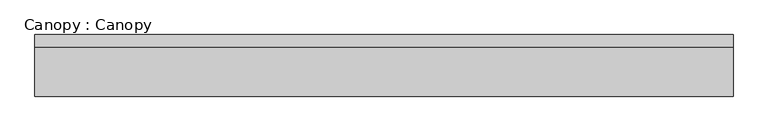
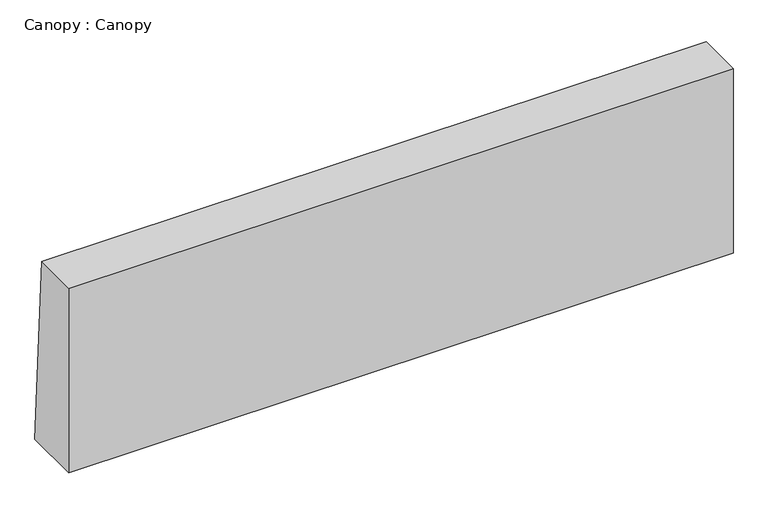
"""IFC4 building model written with IfcOpenShell, lengths in millimetres: proxy geometry, Canopy : Canopy."""

import ifcopenshell
import ifcopenshell.guid

model = None  # the IFC model being written
_history = None  # IfcOwnerHistory: only IFC2X3 demands one
_inside = {}  # id of a spatial element -> (the spatial element, [elements in it])
_under = {}  # id of a project, library or spatial element -> (it, [spatial elements below it])
_declared = {}  # id of a project -> (the project, [libraries it declares])
_typed = {}  # id of a type object -> (the type object, [elements of that type])
_made_of = {}  # id of a material, layer set ... -> (it, [elements and type objects made of it])


def new_model(schema):
    """Start an empty IFC model of exactly this schema.

    Asked for "IFC4X3", IfcOpenShell would pick the latest addendum, in which some entities
    have other attributes; the version numbers below select the first issue.
    IFC2X3 requires an IfcOwnerHistory on every rooted entity: one is made here for all.
    """
    global model, _history
    if schema == "IFC4X3":
        model = ifcopenshell.file(schema_version=(4, 3, 0, 0))
    else:
        model = ifcopenshell.file(schema=schema)
    _inside.clear()
    _under.clear()
    _declared.clear()
    _typed.clear()
    _made_of.clear()
    _history = None
    if model.schema == "IFC2X3":
        org = make("IfcOrganization", Name="unknown")
        user = make(
            "IfcPersonAndOrganization",
            ThePerson=make("IfcPerson", FamilyName="unknown"),
            TheOrganization=org,
        )
        app = make(
            "IfcApplication",
            ApplicationDeveloper=org,
            Version="unknown",
            ApplicationFullName="unknown",
            ApplicationIdentifier="unknown",
        )
        _history = make(
            "IfcOwnerHistory",
            OwningUser=user,
            OwningApplication=app,
            ChangeAction="ADDED",
            CreationDate=0,
        )
    return model


def make(cls, **values):
    """One entity of the class cls with the attributes given. An attribute that is None is left unset."""
    return model.create_entity(
        cls, **{name: value for name, value in values.items() if value is not None}
    )


def rooted(cls, **values):
    """An entity with a GlobalId (a new one), such as an element, a storey or a relation."""
    return make(cls, GlobalId=ifcopenshell.guid.new(), OwnerHistory=_history, **values)


def si_unit(unit_type, name, prefix=None):
    """IfcSIUnit, for example si_unit("LENGTHUNIT", "METRE", prefix="MILLI")."""
    return make("IfcSIUnit", UnitType=unit_type, Prefix=prefix, Name=name)


def assignment(units):
    """IfcUnitAssignment: the units of a project."""
    return None if units is None else make("IfcUnitAssignment", Units=units)


def point(xyz):
    """IfcCartesianPoint."""
    return None if xyz is None else make("IfcCartesianPoint", Coordinates=xyz)


def direction(xyz):
    """IfcDirection."""
    return None if xyz is None else make("IfcDirection", DirectionRatios=xyz)


def frame(location, z_axis=None, x_axis=None):
    """IfcAxis2Placement3D, a coordinate frame: its origin and axes. An axis left out is left unset."""
    return make(
        "IfcAxis2Placement3D",
        Location=point(location),
        Axis=direction(z_axis),
        RefDirection=direction(x_axis),
    )


def origin():
    """The frame at (0, 0, 0) with its axes left unset."""
    return frame((0.0, 0.0, 0.0))


def place(relative_to, where):
    """IfcLocalPlacement: puts the frame where relative to a parent placement (None: the world)."""
    return make(
        "IfcLocalPlacement", PlacementRelTo=relative_to, RelativePlacement=where
    )


def context(
    kind, dimensions, precision=None, world=None, true_north=None, identifier=None
):
    """IfcGeometricRepresentationContext, for example the 3D "Model" context."""
    return make(
        "IfcGeometricRepresentationContext",
        ContextIdentifier=identifier,
        ContextType=kind,
        CoordinateSpaceDimension=dimensions,
        Precision=precision,
        WorldCoordinateSystem=world,
        TrueNorth=true_north,
    )


def project(units=None, contexts=None):
    """IfcProject with its units and contexts."""
    return rooted(
        "IfcProject",
        Name="project",
        RepresentationContexts=contexts,
        UnitsInContext=assignment(units),
    )


def spatial(cls, under=None, at=None, **own):
    """A site, building, storey or space (cls), placed at a placement, below another one or the project."""
    s = rooted(cls, ObjectPlacement=at, **own)
    if under is not None:
        _under.setdefault(under.id(), (under, []))[1].append(s)
    return s


def polyline(points):
    """IfcPolyline through the points."""
    return make("IfcPolyline", Points=[point(p) for p in points])


def outline(outer, holes=None, kind="AREA"):
    """IfcArbitraryClosedProfileDef: a profile drawn as a closed curve; with holes, ...WithVoids."""
    if holes is None:
        return make("IfcArbitraryClosedProfileDef", ProfileType=kind, OuterCurve=outer)
    return make(
        "IfcArbitraryProfileDefWithVoids",
        ProfileType=kind,
        OuterCurve=outer,
        InnerCurves=holes,
    )


def extrude(swept, where, along, depth):
    """IfcExtrudedAreaSolid: the profile swept, set in the frame where, extruded along a direction by depth."""
    return make(
        "IfcExtrudedAreaSolid",
        SweptArea=swept,
        Position=where,
        ExtrudedDirection=direction(along),
        Depth=depth,
    )


def shape(context_of_items, identifier, shape_type, items):
    """IfcShapeRepresentation: the items that make up one representation, for example the "Body"."""
    return make(
        "IfcShapeRepresentation",
        ContextOfItems=context_of_items,
        RepresentationIdentifier=identifier,
        RepresentationType=shape_type,
        Items=items,
    )


def source(mapping_origin, context_of_items, identifier, shape_type, items):
    """IfcRepresentationMap: a shape defined once, which mapped items show again and again."""
    return make(
        "IfcRepresentationMap",
        MappingOrigin=mapping_origin,
        MappedRepresentation=shape(context_of_items, identifier, shape_type, items),
    )


def transform(
    local_origin,
    x_axis=None,
    y_axis=None,
    z_axis=None,
    scale=None,
    scale2=None,
    scale3=None,
    uniform=True,
):
    """IfcCartesianTransformationOperator3D, or its non-uniform kind. x_axis, y_axis, z_axis: its Axis1, 2, 3."""
    if uniform:
        return make(
            "IfcCartesianTransformationOperator3D",
            Axis1=direction(x_axis),
            Axis2=direction(y_axis),
            LocalOrigin=point(local_origin),
            Scale=scale,
            Axis3=direction(z_axis),
        )
    return make(
        "IfcCartesianTransformationOperator3DnonUniform",
        Axis1=direction(x_axis),
        Axis2=direction(y_axis),
        LocalOrigin=point(local_origin),
        Scale=scale,
        Axis3=direction(z_axis),
        Scale2=scale2,
        Scale3=scale3,
    )


def mapped(mapping_source, mapping_target):
    """IfcMappedItem: shows the shape of a source again, moved by a transform."""
    return make(
        "IfcMappedItem", MappingSource=mapping_source, MappingTarget=mapping_target
    )


def made_of(thing, what):
    """Note that an element or type object is made of a material, layer set ...; save() writes the relation."""
    if what is not None:
        _made_of.setdefault(what.id(), (what, []))[1].append(thing)
    return thing


def element(
    cls,
    number,
    at=None,
    inside=None,
    cuts=None,
    type_object=None,
    material=None,
    context=None,
    identifier="Body",
    shape_type=None,
    held_by="IfcProductDefinitionShape",
    body=None,
    shapes=None,
    **own,
):
    """One element of the class cls, such as IfcWall. Its Tag is "e" and its number.

    at: its placement. inside: the storey or other place that contains it. cuts: it is an
    opening in that element (IfcRelVoidsElement). A single representation is given by context,
    identifier, shape_type and body (its items); several are given by shapes. held_by: the class
    of the entity that holds the representations. save() writes the other relations.
    """
    e = rooted(cls, Tag="e%d" % number, ObjectPlacement=at, **own)
    if body is not None:
        shapes = [shape(context, identifier, shape_type, body)]
    if shapes is not None:
        e.Representation = make(held_by, Representations=shapes)
    if inside is not None:
        _inside.setdefault(inside.id(), (inside, []))[1].append(e)
    if cuts is not None:
        rooted(
            "IfcRelVoidsElement", RelatingBuildingElement=cuts, RelatedOpeningElement=e
        )
    if type_object is not None:
        _typed.setdefault(type_object.id(), (type_object, []))[1].append(e)
    return made_of(e, material)


def aggregate(whole, parts):
    """IfcRelAggregates: a whole, such as a stair, and the parts it consists of."""
    return rooted("IfcRelAggregates", RelatingObject=whole, RelatedObjects=parts)


def save(model, path):
    """Write the relations noted so far, then the file.

    IfcRelAggregates (storeys below a building ...), IfcRelContainedInSpatialStructure (elements
    in a storey), IfcRelDefinesByType, IfcRelAssociatesMaterial and IfcRelDeclares: one each for
    every whole, place, type object, material and project.
    """
    for whole, parts in _under.values():
        aggregate(whole, parts)
    for where, things in _inside.values():
        rooted(
            "IfcRelContainedInSpatialStructure",
            RelatedElements=things,
            RelatingStructure=where,
        )
    for kind, things in _typed.values():
        rooted("IfcRelDefinesByType", RelatedObjects=things, RelatingType=kind)
    for what, things in _made_of.values():
        rooted("IfcRelAssociatesMaterial", RelatedObjects=things, RelatingMaterial=what)
    for by, libraries in _declared.values():
        rooted("IfcRelDeclares", RelatingContext=by, RelatedDefinitions=libraries)
    model.write(path)


def canopy_canopy_9389d072(model_context):
    return source(origin(), model_context, "Body", "SweptSolid", [
        extrude(outline(polyline([(150.0, 0.0), (0.0, 0.0), (0.0, 500.0), (120.0, 500.0), (150.0, 0.0)])), frame((-850.0, 0.0, 0.0), z_axis=(1.0, 0.0, 0.0), x_axis=(0.0, 1.0, 0.0)), (0.0, 0.0, 1.0), 1700.0),
    ])


if __name__ == "__main__":
    model = new_model("IFC4")
    model_context = context("Model", 3, world=origin())
    ifc_project = project(units=[si_unit("LENGTHUNIT", "METRE", prefix="MILLI")], contexts=[model_context])
    site = spatial("IfcSite", under=ifc_project)
    building = spatial("IfcBuilding", under=site)
    placement = place(None, origin())
    canopy_canopy_shape = canopy_canopy_9389d072(model_context)
    element("IfcBuildingElementProxy", 1, Name="Canopy : Canopy", ObjectType="Canopy : Canopy", at=placement, inside=building, context=model_context, shape_type="MappedRepresentation", body=[
        mapped(canopy_canopy_shape, transform((0.0, 0.0, 0.0), x_axis=(1.0, 0.0, 0.0), y_axis=(0.0, 1.0, 0.0), z_axis=(0.0, 0.0, 1.0))),
    ])
    save(model, "model.ifc")

# Revit data of these elements
# Type "Canopy : Canopy"
#   Type Comments = "CV-AG"
#   H_Rebar Ratio = 0.1
#   Canopy Width [instance default] = 1700 mm
#   Canopy Length [instance default] = 1000 mm
#   Canopy L.P = 120 mm
#   Canopy H.P = 150 mm
#   구조재료 = Concrete_f'c=28MPa(Cylender)
#   Default Elevation = 0
# Element 1 (IfcBuildingElementProxy, "Canopy : Canopy")
#   Canopy Length = 500 mm
#   Materials on its faces: "Concrete_f'c=28MPa(Cylender)"
# Materials
#   "Concrete_f'c=28MPa(Cylender)": class "Concrete", colour RGB 176 176 176, transparency 0, Description = "Reinf. Conc.", Cost = 0, Image = Concrete.Cast-In-Place.Flat.Polished.Grey.jpg
